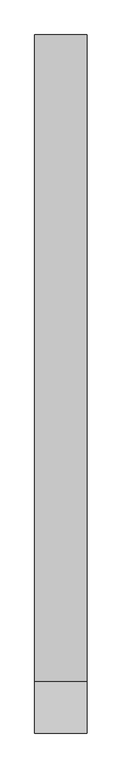
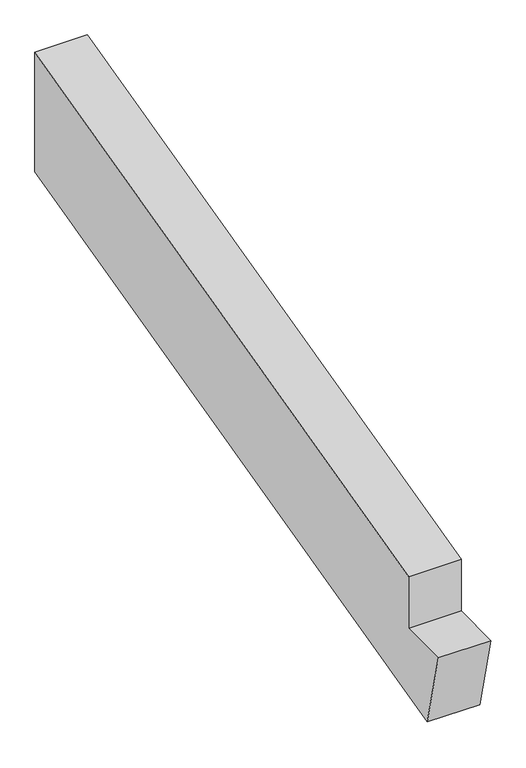
"""IFC4 building model written with IfcOpenShell, lengths in millimetres: proxy geometry, Framing8:Framing024:286352 : Framing8:Framing024:286352."""

from ifc_helpers import new_model, si_unit, frame, origin, place, context, project, spatial, polyline, outline, extrude, source, transform, mapped, element, save


def generic_models_093dd6d1(model_context):
    return source(origin(), model_context, "Body", "SweptSolid", [
        extrude(outline(polyline([(-5040.1231329, 42411.3663805), (-5096.6420486, 42642.0307603), (-4946.0750638, 42642.0307603), (-4946.0750638, 42800.8143799), (-3066.3240751, 43270.717426), (-3066.3240751, 42903.8818003), (-5040.1231329, 42411.3663805)])), frame((18311.909108, 0.0, 0.0), z_axis=(1.0, 0.0, 0.0), x_axis=(0.0, 1.0, 0.0)), (0.0, 0.0, 1.0), 152.4),
    ])


if __name__ == "__main__":
    model = new_model("IFC4")
    model_context = context("Model", 3, world=origin())
    ifc_project = project(units=[si_unit("LENGTHUNIT", "METRE", prefix="MILLI")], contexts=[model_context])
    site = spatial("IfcSite", under=ifc_project)
    building = spatial("IfcBuilding", under=site)
    placement = place(None, origin())
    generic_models_shape = generic_models_093dd6d1(model_context)
    element("IfcBuildingElementProxy", 1, Name="Framing8:Framing024:286352 : Framing8:Framing024:286352", ObjectType="Framing8:Framing024:286352 : Framing8:Framing024:286352", at=placement, inside=building, context=model_context, shape_type="MappedRepresentation", body=[
        mapped(generic_models_shape, transform((0.0, 0.0, 0.0), x_axis=(1.0, 0.0, 0.0), y_axis=(0.0, 1.0, 0.0), z_axis=(0.0, 0.0, 1.0))),
    ])
    save(model, "model.ifc")

# Revit data of these elements
# Type "Framing8:Framing024:286352 : Framing8:Framing024:286352"
#   NameOverride = "Framing8:Framing024:286352"
#   ObjectTypeOverride = "Framing8:Framing024"
#   Reference = "Framing024"
#   Category = "Generic Models"
#   Tag = "286352"
# Element 1 (IfcBuildingElementProxy, "Framing8:Framing024:286352 : Framing8:Framing024:286352")
#   Materials on its faces: "WOOD FRAMING (SEE STRUCT DWGS)"
# Materials
#   "WOOD FRAMING (SEE STRUCT DWGS)": class "Unassigned", colour RGB 224 188 168, transparency 0, Cost = 0
